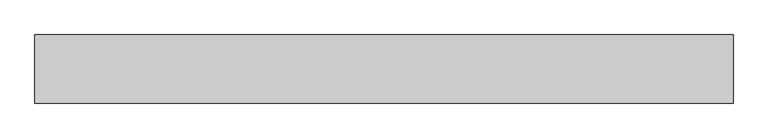
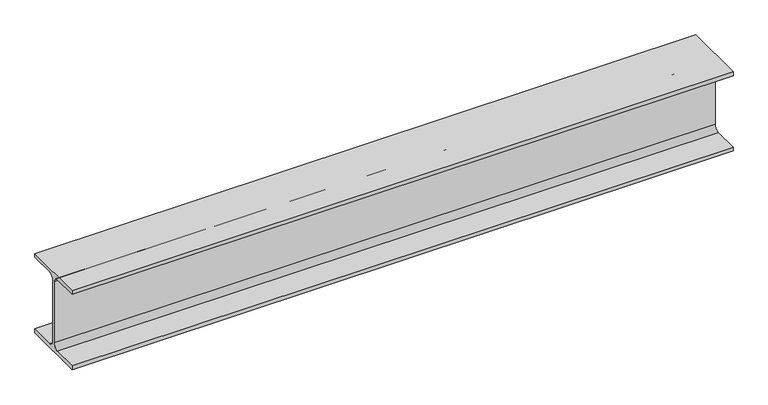
"""IFC4 building model written with IfcOpenShell, lengths in millimetres: beam geometry, 0912_Steel Framing_H-KSD3502 : H_SB_ASB_H-194x150x6x9."""

from ifc_helpers import new_model, si_unit, point, frame, frame_2d, origin, place, context, project, spatial, polyline, circle_curve, trimmed, segment, composite_curve, outline, extrude, source, transform, mapped, element, save


def beam_7cd79bbf(model_context):
    return source(origin(), model_context, "Body", "SweptSolid", [
        extrude(outline(composite_curve([segment(polyline([(-75.0, -88.0), (-16.0, -88.0)]), True, "CONTINUOUS"), segment(trimmed(circle_curve(frame_2d((-16.0, -75.0)), 13.0), [point((-16.0, -88.0))], [point((-3.0, -75.0))], True, "CARTESIAN"), True, "CONTINUOUS"), segment(polyline([(-3.0, -75.0), (-3.0, 75.0)]), True, "CONTINUOUS"), segment(trimmed(circle_curve(frame_2d((-16.0, 75.0)), 13.0), [point((-3.0, 75.0))], [point((-16.0, 88.0))], True, "CARTESIAN"), True, "CONTINUOUS"), segment(polyline([(-16.0, 88.0), (-75.0, 88.0), (-75.0, 97.0), (75.0, 97.0), (75.0, 88.0), (16.0, 88.0)]), True, "CONTINUOUS"), segment(trimmed(circle_curve(frame_2d((16.0, 75.0)), 13.0), [point((16.0, 88.0))], [point((3.0, 75.0))], True, "CARTESIAN"), True, "CONTINUOUS"), segment(polyline([(3.0, 75.0), (3.0, -75.0)]), True, "CONTINUOUS"), segment(trimmed(circle_curve(frame_2d((16.0, -75.0)), 13.0), [point((3.0, -75.0))], [point((16.0, -88.0))], True, "CARTESIAN"), True, "CONTINUOUS"), segment(polyline([(16.0, -88.0), (75.0, -88.0), (75.0, -97.0), (-75.0, -97.0), (-75.0, -88.0)]), True, "CONTINUOUS")], self_intersect=False)), frame((-549.6452709, 0.0, 0.0), z_axis=(1.0, 0.0, 0.0), x_axis=(0.0, 1.0, 0.0)), (0.0, 0.0, 1.0), 1537.9998794),
    ])


if __name__ == "__main__":
    model = new_model("IFC4")
    model_context = context("Model", 3, world=origin())
    ifc_project = project(units=[si_unit("LENGTHUNIT", "METRE", prefix="MILLI")], contexts=[model_context])
    site = spatial("IfcSite", under=ifc_project)
    building = spatial("IfcBuilding", under=site)
    placement = place(None, origin())
    beam_shape = beam_7cd79bbf(model_context)
    element("IfcBeam", 1, ObjectType="0912_Steel Framing_H-KSD3502 : H_SB_ASB_H-194x150x6x9", at=placement, inside=building, context=model_context, shape_type="MappedRepresentation", body=[
        mapped(beam_shape, transform((0.0, 0.0, 0.0), x_axis=(1.0, 0.0, 0.0), y_axis=(0.0, 1.0, 0.0), z_axis=(0.0, 0.0, 1.0))),
    ])
    save(model, "model.ifc")

# Revit data of these elements
# Type "0912_Steel Framing_H-KSD3502 : H_SB_ASB_H-194x150x6x9"
#   H_WM Code_1 = "S01AA002-00001 | Main Steel Structure Fabrication Work | Shelter/Building | Medium Steel - Standard (90KG/M>Weight≥30KG/M) | Material: (   )"
#   H_WM Code_2 = "S03AA028-00001 | Main Steel Structure Erection Work | Shelter/Building | Medium Steel (90KG/M>Weight≥30KG/M) | Material: (   )"
#   H_WM Code_3 = "S01AA010-00001 | Main Steel Structure Fabrication Work | Shelter/Building | Steel Painting/Coating | for Non-Fireproofed Steel Surface, Surface Preparation, Primer, Second & Final Coat | Material: (   )"
#   H_Q'ty Cal Type Tag = "SB-Q2"
#   Width = 15.0 cm
#   Web Thickness = 0.6 cm
#   Web Fillet = 1.3 cm
#   Warping Constant = 43316.0 cm⁶
#   W = 0
#   Torsional Moment of Inertia = 8.622 cm⁴
#   Section Area = 39.01 cm²
#   Plastic Modulus weak axis = 104.0 cm³
#   Plastic Modulus strong axis = 309.0 cm³
#   Perimeter = 0.95 m²/m
#   Nominal Weight = 30.60 kgf/m
#   Moment of Inertia weak axis = 507.00 cm⁴
#   Moment of Inertia strong axis = 2690.00 cm⁴
#   Height = 19.4 cm
#   Flange Thickness = 0.9 cm
#   Elastic Modulus weak axis = 67.6 cm³
#   Elastic Modulus strong axis = 277.0 cm³
#   Centroid Vertical = 9.7 cm
#   Centroid Horizontal = 7.5 cm
#   Ix = 26900000
#   Length [instance default] = 1.5240 m
#   Zx = 309000
#   b = 0.1500 m
#   h = 0.1940 m
#   r = 0.0130 m
#   s = 0.0060 m
#   t = 0.0090 m
#   A = 0.003901 m²
#   Structural Material [instance default] = Steel, 45-345
#   Assembly Code = ""
# Element 1 (IfcBeam, "0912_Steel Framing_H-KSD3502 : H_SB_ASB_H-194x150x6x9")
#   Structural Material = none
# Materials
#   "Steel, 45-345": class "Metal", colour RGB 189 187 185, transparency 0, Description = "Steel 345 MPa", Cost = 0
